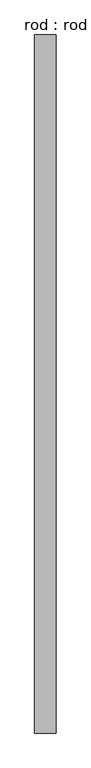
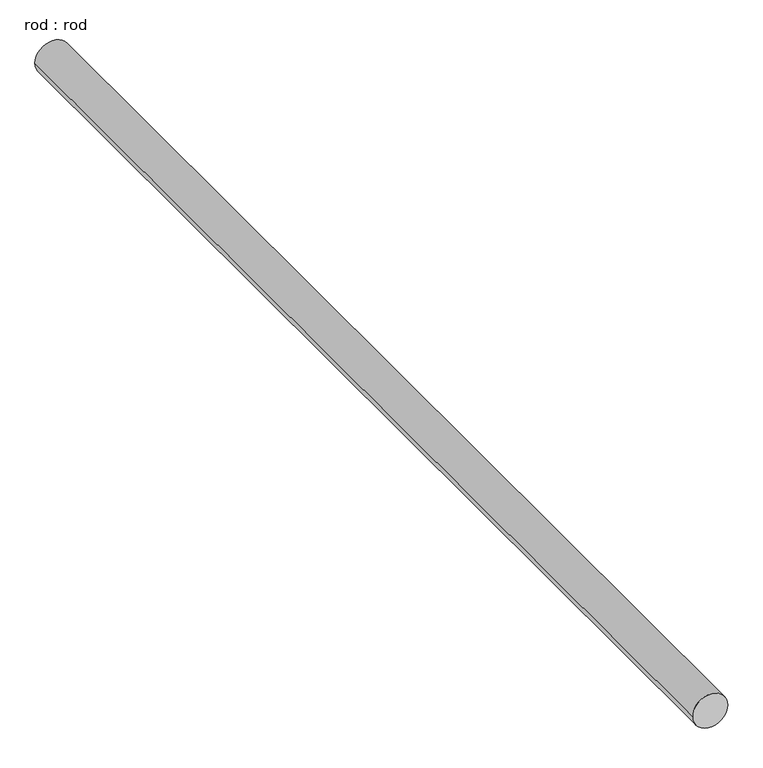
"""IFC4 building model written with IfcOpenShell, lengths in millimetres: proxy geometry, rod : rod."""

from ifc_helpers import new_model, si_unit, point, frame, frame_2d, origin, place, context, project, spatial, circle_curve, trimmed, segment, composite_curve, outline, extrude, source, transform, mapped, element, save


def rod_rod_0ecd3f0c(model_context):
    return source(origin(), model_context, "Body", "SweptSolid", [
        extrude(outline(composite_curve([segment(trimmed(circle_curve(frame_2d((0.0108462, 0.0)), 200.0), [point((0.0108462, 200.0))], [point((0.0108462, -200.0))], False, "CARTESIAN"), True, "CONTINUOUS"), segment(trimmed(circle_curve(frame_2d((0.0108462, 0.0)), 200.0), [point((0.0108462, -200.0))], [point((0.0108462, 200.0))], False, "CARTESIAN"), True, "CONTINUOUS")], self_intersect=False)), frame((0.0, -2407.2713847, 0.0), z_axis=(0.0, 1.0, 0.0), x_axis=(0.0, 0.0, 1.0)), (0.0, 0.0, 1.0), 13000.0),
    ])


if __name__ == "__main__":
    model = new_model("IFC4")
    model_context = context("Model", 3, world=origin())
    ifc_project = project(units=[si_unit("LENGTHUNIT", "METRE", prefix="MILLI")], contexts=[model_context])
    site = spatial("IfcSite", under=ifc_project)
    building = spatial("IfcBuilding", under=site)
    placement = place(None, origin())
    rod_rod_shape = rod_rod_0ecd3f0c(model_context)
    element("IfcBuildingElementProxy", 1, Name="rod : rod", ObjectType="rod : rod", at=placement, inside=building, context=model_context, shape_type="MappedRepresentation", body=[
        mapped(rod_rod_shape, transform((0.0, 0.0, 0.0), x_axis=(1.0, 0.0, 0.0), y_axis=(0.0, 1.0, 0.0), z_axis=(0.0, 0.0, 1.0))),
    ])
    save(model, "model.ifc")

# Revit data of these elements
# Type "rod : rod"
#   Default Elevation = 0
